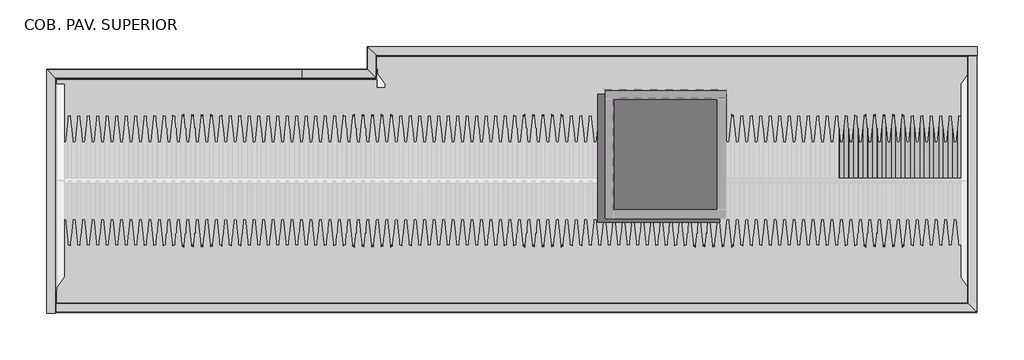
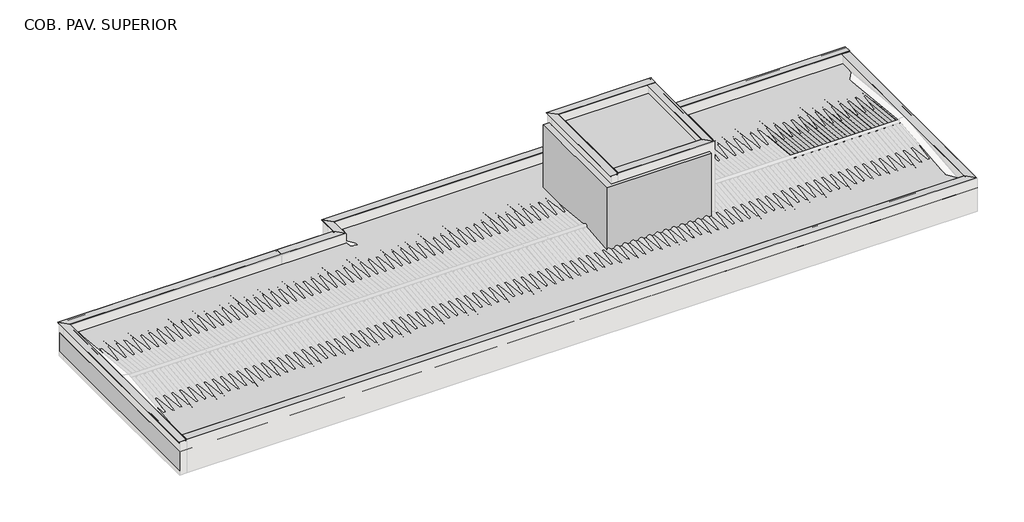
# One storey, part 8 of 8: 25 beams, 7 columns, 4 proxies.
# Revit data of these elements (continued)
# Elements 1, 2, 3, 4, 5, 6 (IfcBeam, "Madeira de lei : Berço 6x12cm")
#   Comments = ""
#   Uso = "TELHADOS ESTRUTURAS"
#   Compr Cmcl = 6.00 m
#   Structural Material = .MADEIRAMENTO
#   Phase Created = CC_AP
#   Materials on its faces: ".MADEIRAMENTO"
# Elements 7, 8 (IfcBeam, "Madeira de lei : Berço 6x12cm")
#   Comments = ""
#   Uso = "TELHADOS ESTRUTURAS"
#   Compr Cmcl = 1.00 m
#   Structural Material = .MADEIRAMENTO
#   Phase Created = CC_AP
#   Materials on its faces: ".MADEIRAMENTO"
# Element 9 (IfcBeam, "Madeira de lei : Berço 6x12cm")
#   Comments = ""
#   Uso = "TELHADOS ESTRUTURAS"
#   Compr Cmcl = 3.00 m
#   Structural Material = .MADEIRAMENTO
#   Phase Created = CC_AP
#   Materials on its faces: ".MADEIRAMENTO"
# Elements 10, 11, 12, 13, 14, 15, 16, 17, 18, 19, 20, 21, 22, 23, 24, 25 (IfcBeam, "Telha Ondulada : Fibrocimento")
#   Uso = "TELHADOS TELHAS"
#   Phase Created = CC_AP
#   Materials on its faces: ".TELHA DE FIBROCIMENTO"
# Element 26 (IfcBuildingElementProxy, "VOLUME DA CAIXA D'ÁGUA : VOLUME DA CAIXA D'ÁGUA")
#   Phase Created = CC_EV
#   Materials on its faces: "Forma padrão"
# Element 27 (IfcBuildingElementProxy, ".CC_RUFO_PINGADEIRA_22 cm")
#   Uso = "TELHADOS RUFOS"
#   Nível de Ref. = "SUPERIOR"
#   Phase Created = CC_AP
#   Materials on its faces: ".ALUMÍNIO COM PINTURA LÁTEX BRANCA"
# Element 28 (IfcBuildingElementProxy, ".CC_RUFO_PINGADEIRA_22 cm")
#   Uso = "TELHADOS RUFOS"
#   Nível de Ref. = "MURO"
#   Phase Created = CC_AP
#   Materials on its faces: ".ALUMÍNIO COM PINTURA LÁTEX BRANCA"
# Element 29 (IfcBuildingElementProxy, "COBERTURA PAVIMENTO SUPERIOR : COBERTURA PAVIMENTO SUPERIOR")
#   Phase Created = CC_EV
#   Materials on its faces: "Forma padrão"
# Element 30 (IfcColumn, "Madeira de lei-Coluna : Pontalete 6X16cm")
#   Comments = ""
#   Uso = "TELHADOS ESTRUTURAS"
#   Compr Cmcl = 6.00 m
#   Structural Material = .MADEIRAMENTO
#   Phase Created = CC_AP
#   Materials on its faces: ".MADEIRAMENTO"
# Elements 31, 32 (IfcColumn, "Madeira de lei-Coluna : Pontalete 6X16cm")
#   Comments = ""
#   Uso = "TELHADOS ESTRUTURAS"
#   Compr Cmcl = 4.00 m
#   Structural Material = .MADEIRAMENTO
#   Phase Created = CC_AP
#   Materials on its faces: ".MADEIRAMENTO"
# Elements 33, 34, 35, 36 (IfcColumn, "Madeira de lei-Coluna : Pontalete 6X16cm")
#   Comments = ""
#   Uso = "TELHADOS ESTRUTURAS"
#   Compr Cmcl = 5.00 m
#   Structural Material = .MADEIRAMENTO
#   Phase Created = CC_AP
#   Materials on its faces: ".MADEIRAMENTO"
# Materials
#   ".TELHA DE FIBROCIMENTO": class "CC_TELHADO", colour RGB 77 77 76, transparency 0, Description = "TELHA ONDULADA FIBROCIMENTO", Cost = 0
#   ".MADEIRAMENTO": class ".CC_MADEIRAS", colour RGB 212 179 113, transparency 0, Cost = 0
#   "Forma padrão": class "Genérico", colour RGB 185 189 196, transparency 0.5, Cost = 0
#   ".ALUMÍNIO COM PINTURA LÁTEX BRANCA": class "Generic", colour RGB 250 250 250, transparency 0, Cost = 0
